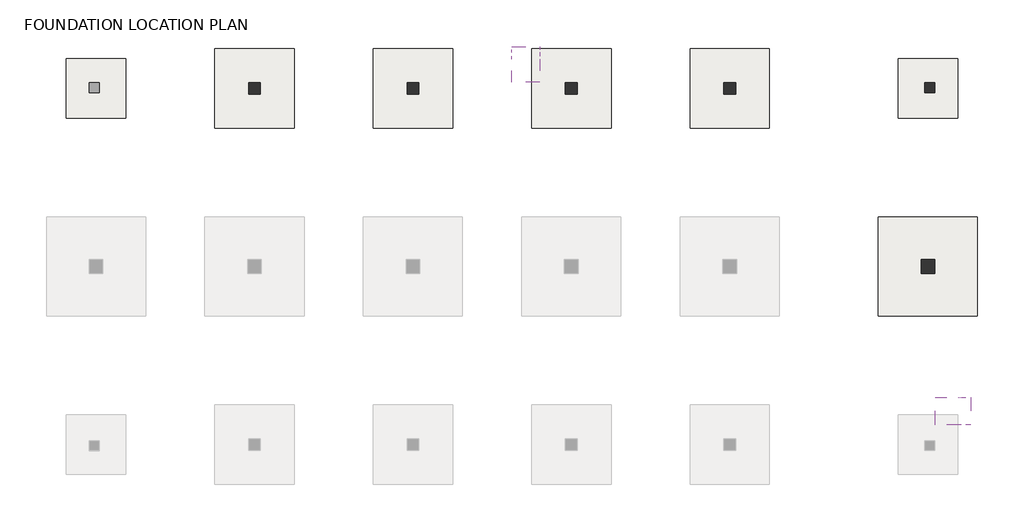
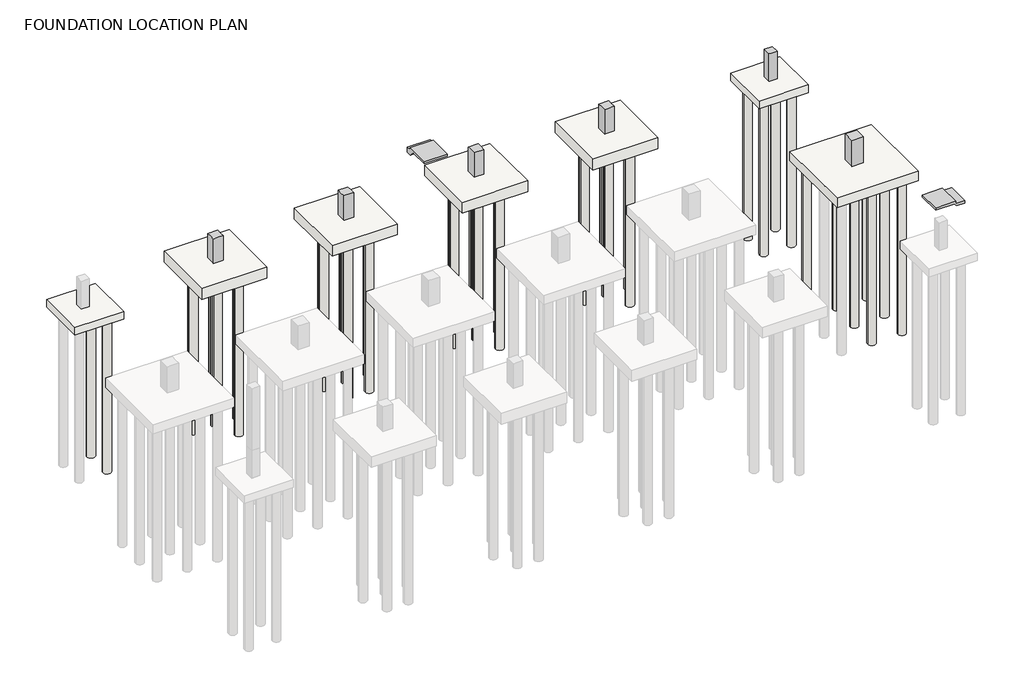
# One storey, part 3 of 3: 48 slabs, 6 columns, 2 proxies.
"""IFC4 building model written with IfcOpenShell, lengths in millimetres."""

import ifcopenshell
import ifcopenshell.guid

model = None  # the IFC model being written
_history = None  # IfcOwnerHistory: only IFC2X3 demands one
_inside = {}  # id of a spatial element -> (the spatial element, [elements in it])
_under = {}  # id of a project, library or spatial element -> (it, [spatial elements below it])
_declared = {}  # id of a project -> (the project, [libraries it declares])
_typed = {}  # id of a type object -> (the type object, [elements of that type])
_made_of = {}  # id of a material, layer set ... -> (it, [elements and type objects made of it])


def new_model(schema):
    """Start an empty IFC model of exactly this schema.

    Asked for "IFC4X3", IfcOpenShell would pick the latest addendum, in which some entities
    have other attributes; the version numbers below select the first issue.
    IFC2X3 requires an IfcOwnerHistory on every rooted entity: one is made here for all.
    """
    global model, _history
    if schema == "IFC4X3":
        model = ifcopenshell.file(schema_version=(4, 3, 0, 0))
    else:
        model = ifcopenshell.file(schema=schema)
    _inside.clear()
    _under.clear()
    _declared.clear()
    _typed.clear()
    _made_of.clear()
    _history = None
    if model.schema == "IFC2X3":
        org = make("IfcOrganization", Name="unknown")
        user = make(
            "IfcPersonAndOrganization",
            ThePerson=make("IfcPerson", FamilyName="unknown"),
            TheOrganization=org,
        )
        app = make(
            "IfcApplication",
            ApplicationDeveloper=org,
            Version="unknown",
            ApplicationFullName="unknown",
            ApplicationIdentifier="unknown",
        )
        _history = make(
            "IfcOwnerHistory",
            OwningUser=user,
            OwningApplication=app,
            ChangeAction="ADDED",
            CreationDate=0,
        )
    return model


def make(cls, **values):
    """One entity of the class cls with the attributes given. An attribute that is None is left unset."""
    return model.create_entity(
        cls, **{name: value for name, value in values.items() if value is not None}
    )


def rooted(cls, **values):
    """An entity with a GlobalId (a new one), such as an element, a storey or a relation."""
    return make(cls, GlobalId=ifcopenshell.guid.new(), OwnerHistory=_history, **values)


def si_unit(unit_type, name, prefix=None):
    """IfcSIUnit, for example si_unit("LENGTHUNIT", "METRE", prefix="MILLI")."""
    return make("IfcSIUnit", UnitType=unit_type, Prefix=prefix, Name=name)


def assignment(units):
    """IfcUnitAssignment: the units of a project."""
    return None if units is None else make("IfcUnitAssignment", Units=units)


def point(xyz):
    """IfcCartesianPoint."""
    return None if xyz is None else make("IfcCartesianPoint", Coordinates=xyz)


def direction(xyz):
    """IfcDirection."""
    return None if xyz is None else make("IfcDirection", DirectionRatios=xyz)


def frame(location, z_axis=None, x_axis=None):
    """IfcAxis2Placement3D, a coordinate frame: its origin and axes. An axis left out is left unset."""
    return make(
        "IfcAxis2Placement3D",
        Location=point(location),
        Axis=direction(z_axis),
        RefDirection=direction(x_axis),
    )


def frame_2d(location, x_axis=None):
    """IfcAxis2Placement2D, a coordinate frame in the plane: its origin and x axis."""
    return make(
        "IfcAxis2Placement2D", Location=point(location), RefDirection=direction(x_axis)
    )


def origin():
    """The frame at (0, 0, 0) with its axes left unset."""
    return frame((0.0, 0.0, 0.0))


def place(relative_to, where):
    """IfcLocalPlacement: puts the frame where relative to a parent placement (None: the world)."""
    return make(
        "IfcLocalPlacement", PlacementRelTo=relative_to, RelativePlacement=where
    )


def context(
    kind, dimensions, precision=None, world=None, true_north=None, identifier=None
):
    """IfcGeometricRepresentationContext, for example the 3D "Model" context."""
    return make(
        "IfcGeometricRepresentationContext",
        ContextIdentifier=identifier,
        ContextType=kind,
        CoordinateSpaceDimension=dimensions,
        Precision=precision,
        WorldCoordinateSystem=world,
        TrueNorth=true_north,
    )


def project(units=None, contexts=None):
    """IfcProject with its units and contexts."""
    return rooted(
        "IfcProject",
        Name="project",
        RepresentationContexts=contexts,
        UnitsInContext=assignment(units),
    )


def spatial(cls, under=None, at=None, **own):
    """A site, building, storey or space (cls), placed at a placement, below another one or the project."""
    s = rooted(cls, ObjectPlacement=at, **own)
    if under is not None:
        _under.setdefault(under.id(), (under, []))[1].append(s)
    return s


def polyline(points):
    """IfcPolyline through the points."""
    return make("IfcPolyline", Points=[point(p) for p in points])


def circle_curve(where, radius):
    """IfcCircle in the frame where."""
    return make("IfcCircle", Position=where, Radius=radius)


def trimmed(basis, trim1, trim2, sense, master):
    """IfcTrimmedCurve: the piece of a basis curve between two trims."""
    return make(
        "IfcTrimmedCurve",
        BasisCurve=basis,
        Trim1=trim1,
        Trim2=trim2,
        SenseAgreement=sense,
        MasterRepresentation=master,
    )


def segment(curve, same_sense, transition):
    """IfcCompositeCurveSegment."""
    return make(
        "IfcCompositeCurveSegment",
        Transition=transition,
        SameSense=same_sense,
        ParentCurve=curve,
    )


def composite_curve(segments, self_intersect=None):
    """IfcCompositeCurve: segments joined end to end."""
    return make("IfcCompositeCurve", Segments=segments, SelfIntersect=self_intersect)


def outline(outer, holes=None, kind="AREA"):
    """IfcArbitraryClosedProfileDef: a profile drawn as a closed curve; with holes, ...WithVoids."""
    if holes is None:
        return make("IfcArbitraryClosedProfileDef", ProfileType=kind, OuterCurve=outer)
    return make(
        "IfcArbitraryProfileDefWithVoids",
        ProfileType=kind,
        OuterCurve=outer,
        InnerCurves=holes,
    )


def extrude(swept, where, along, depth):
    """IfcExtrudedAreaSolid: the profile swept, set in the frame where, extruded along a direction by depth."""
    return make(
        "IfcExtrudedAreaSolid",
        SweptArea=swept,
        Position=where,
        ExtrudedDirection=direction(along),
        Depth=depth,
    )


def faces_of(points, faces, orient=None, outer=None):
    """IfcFace entities. A face is a list of loops; a loop is a list of indices into points, from 0.

    orient and outer hold one flag for each loop. By default every Orientation is true, the
    first loop of a face is its IfcFaceOuterBound and the others are IfcFaceBound.
    """
    made = []
    for i, loops in enumerate(faces):
        bounds = []
        for j, loop in enumerate(loops):
            is_outer = j == 0 if outer is None else outer[i][j]
            bounds.append(
                make(
                    "IfcFaceOuterBound" if is_outer else "IfcFaceBound",
                    Bound=make("IfcPolyLoop", Polygon=[points[k] for k in loop]),
                    Orientation=True if orient is None else orient[i][j],
                )
            )
        made.append(make("IfcFace", Bounds=bounds))
    return made


def faceted_brep(points, faces, orient=None, outer=None, voids=None):
    """IfcFacetedBrep: a solid bounded by flat faces; with voids (closed shells), ...WithVoids."""
    shared = [point(p) for p in points]
    hull = make("IfcClosedShell", CfsFaces=faces_of(shared, faces, orient, outer))
    if voids is None:
        return make("IfcFacetedBrep", Outer=hull)
    return make(
        "IfcFacetedBrepWithVoids",
        Outer=hull,
        Voids=[
            make(cls, CfsFaces=faces_of(shared, fs, o, b)) for cls, fs, o, b in voids
        ],
    )


def shape(context_of_items, identifier, shape_type, items):
    """IfcShapeRepresentation: the items that make up one representation, for example the "Body"."""
    return make(
        "IfcShapeRepresentation",
        ContextOfItems=context_of_items,
        RepresentationIdentifier=identifier,
        RepresentationType=shape_type,
        Items=items,
    )


def source(mapping_origin, context_of_items, identifier, shape_type, items):
    """IfcRepresentationMap: a shape defined once, which mapped items show again and again."""
    return make(
        "IfcRepresentationMap",
        MappingOrigin=mapping_origin,
        MappedRepresentation=shape(context_of_items, identifier, shape_type, items),
    )


def transform(
    local_origin,
    x_axis=None,
    y_axis=None,
    z_axis=None,
    scale=None,
    scale2=None,
    scale3=None,
    uniform=True,
):
    """IfcCartesianTransformationOperator3D, or its non-uniform kind. x_axis, y_axis, z_axis: its Axis1, 2, 3."""
    if uniform:
        return make(
            "IfcCartesianTransformationOperator3D",
            Axis1=direction(x_axis),
            Axis2=direction(y_axis),
            LocalOrigin=point(local_origin),
            Scale=scale,
            Axis3=direction(z_axis),
        )
    return make(
        "IfcCartesianTransformationOperator3DnonUniform",
        Axis1=direction(x_axis),
        Axis2=direction(y_axis),
        LocalOrigin=point(local_origin),
        Scale=scale,
        Axis3=direction(z_axis),
        Scale2=scale2,
        Scale3=scale3,
    )


def mapped(mapping_source, mapping_target):
    """IfcMappedItem: shows the shape of a source again, moved by a transform."""
    return make(
        "IfcMappedItem", MappingSource=mapping_source, MappingTarget=mapping_target
    )


def made_of(thing, what):
    """Note that an element or type object is made of a material, layer set ...; save() writes the relation."""
    if what is not None:
        _made_of.setdefault(what.id(), (what, []))[1].append(thing)
    return thing


def element(
    cls,
    number,
    at=None,
    inside=None,
    cuts=None,
    type_object=None,
    material=None,
    context=None,
    identifier="Body",
    shape_type=None,
    held_by="IfcProductDefinitionShape",
    body=None,
    shapes=None,
    **own,
):
    """One element of the class cls, such as IfcWall. Its Tag is "e" and its number.

    at: its placement. inside: the storey or other place that contains it. cuts: it is an
    opening in that element (IfcRelVoidsElement). A single representation is given by context,
    identifier, shape_type and body (its items); several are given by shapes. held_by: the class
    of the entity that holds the representations. save() writes the other relations.
    """
    e = rooted(cls, Tag="e%d" % number, ObjectPlacement=at, **own)
    if body is not None:
        shapes = [shape(context, identifier, shape_type, body)]
    if shapes is not None:
        e.Representation = make(held_by, Representations=shapes)
    if inside is not None:
        _inside.setdefault(inside.id(), (inside, []))[1].append(e)
    if cuts is not None:
        rooted(
            "IfcRelVoidsElement", RelatingBuildingElement=cuts, RelatedOpeningElement=e
        )
    if type_object is not None:
        _typed.setdefault(type_object.id(), (type_object, []))[1].append(e)
    return made_of(e, material)


def aggregate(whole, parts):
    """IfcRelAggregates: a whole, such as a stair, and the parts it consists of."""
    return rooted("IfcRelAggregates", RelatingObject=whole, RelatedObjects=parts)


def save(model, path):
    """Write the relations noted so far, then the file.

    IfcRelAggregates (storeys below a building ...), IfcRelContainedInSpatialStructure (elements
    in a storey), IfcRelDefinesByType, IfcRelAssociatesMaterial and IfcRelDeclares: one each for
    every whole, place, type object, material and project.
    """
    for whole, parts in _under.values():
        aggregate(whole, parts)
    for where, things in _inside.values():
        rooted(
            "IfcRelContainedInSpatialStructure",
            RelatedElements=things,
            RelatingStructure=where,
        )
    for kind, things in _typed.values():
        rooted("IfcRelDefinesByType", RelatedObjects=things, RelatingType=kind)
    for what, things in _made_of.values():
        rooted("IfcRelAssociatesMaterial", RelatedObjects=things, RelatingMaterial=what)
    for by, libraries in _declared.values():
        rooted("IfcRelDeclares", RelatingContext=by, RelatedDefinitions=libraries)
    model.write(path)


def generic_models_a06d278e(model_context):
    return source(origin(), model_context, "Body", "SweptSolid", [
        extrude(outline(polyline([(599.905241, 43602.1335861), (599.905241, 42370.0), (449.905241, 42370.0), (449.905241, 43520.0), (299.905241, 43670.0), (299.905241, 44170.4893475), (449.905241, 44170.4893475), (449.905241, 43602.1335861), (599.905241, 43602.1335861)])), frame((0.0, 21999.5208589, 0.0), z_axis=(0.0, 1.0, 0.0), x_axis=(0.0, 0.0, 1.0)), (0.0, 0.0, 1.0), 1400.0),
    ])


def generic_models_c40cd3bd(model_context):
    return source(origin(), model_context, "Body", "SweptSolid", [
        extrude(outline(polyline([(40819.5208589, 599.905241), (40819.5208589, 449.905241), (41119.5208589, 449.905241), (41119.5208589, 109.2314637), (40810.1946362, 109.2314637), (40469.5208589, 449.905241), (39319.5208589, 449.905241), (39319.5208589, 599.905241), (40819.5208589, 599.905241)])), frame((21000.0, 0.0, 0.0), z_axis=(1.0, 0.0, 0.0), x_axis=(0.0, 1.0, 0.0)), (0.0, 0.0, 1.0), 1400.0),
    ])


model = new_model("IFC4")

# Units and contexts
model_context = context("Model", 3, world=origin())
ifc_project = project(units=[si_unit("LENGTHUNIT", "METRE", prefix="MILLI")], contexts=[model_context])

# Site, building, storey
site = spatial("IfcSite", under=ifc_project)
building = spatial("IfcBuilding", under=site)
storey = spatial("IfcBuildingStorey", under=building, Name="FOUNDATION LOCATION PLAN", Elevation=-1699.994759)

# Proxies
placement = place(None, origin())
generic_models_shape = generic_models_a06d278e(model_context)
element("IfcBuildingElementProxy", 1, Name="벽 5 : 벽 1", ObjectType="벽 5 : 벽 1", at=placement, inside=storey, context=model_context, shape_type="MappedRepresentation", body=[
    mapped(generic_models_shape, transform((0.0, 0.0, 0.0), x_axis=(1.0, 0.0, 0.0), y_axis=(0.0, 1.0, 0.0), z_axis=(0.0, 0.0, 1.0))),
])
generic_models_2_shape = generic_models_c40cd3bd(model_context)
element("IfcBuildingElementProxy", 2, Name="벽 1 : 벽 1", ObjectType="벽 1 : 벽 1", at=placement, inside=storey, context=model_context, shape_type="MappedRepresentation", body=[
    mapped(generic_models_2_shape, transform((0.0, 0.0, 0.0), x_axis=(1.0, 0.0, 0.0), y_axis=(0.0, 1.0, 0.0), z_axis=(0.0, 0.0, 1.0))),
])

# Columns
element("IfcColumn", 3, ObjectType="Concrete-Rectangular-Column_R1 : CLS111_RC COLUMN_UG_C1", at=placement, inside=storey, context=model_context, shape_type="Brep", body=[
    faceted_brep([(41850.0, 39299.5208589, -1199.994759), (42350.0, 39299.5208589, -1199.994759), (42350.0, 38799.5208589, -1199.994759), (41850.0, 38799.5208589, -1199.994759), (41850.0, 39299.5208589, 600.005241), (42350.0, 39299.5208589, 600.005241), (41850.0, 38799.5208589, 450.005241), (41850.0, 38799.5208589, 600.005241), (41850.0, 38999.7368538, 600.005241), (42350.0, 38799.5208589, 600.005241), (42000.0, 38799.5208589, 600.005241)], [[[0, 1, 2, 3]], [[1, 0, 4, 5]], [[0, 3, 6, 7, 8, 4]], [[3, 2, 9, 10, 7, 6]], [[2, 1, 5, 9]], [[5, 4, 8, 7, 10, 9]]]),
])
element("IfcColumn", 4, ObjectType="Concrete-Rectangular-Column_R1 : CLS111_RC COLUMN_UG_C3", at=placement, inside=storey, context=model_context, shape_type="Brep", body=[
    faceted_brep([(41650.0, 30349.5208589, -1099.994759), (42350.0, 30349.5208589, -1099.994759), (42350.0, 29649.5208589, -1099.994759), (41650.0, 29649.5208589, -1099.994759), (41650.0, 30349.5208589, 450.005241), (41650.0, 30349.5208589, 600.005241), (42000.0, 30349.5208589, 600.005241), (42350.0, 30349.5208589, 600.005241), (41650.0, 29649.5208589, 450.005241), (41650.0, 29649.5208589, 600.005241), (42350.0, 29649.5208589, 600.005241)], [[[0, 1, 2, 3]], [[1, 0, 4, 5, 6, 7]], [[0, 3, 8, 9, 5, 4]], [[3, 2, 10, 9, 8]], [[2, 1, 7, 10]], [[5, 9, 10, 7, 6]]]),
])
element("IfcColumn", 5, ObjectType="Concrete-Rectangular-Column_R1 : CLS111_RC COLUMN_UG_C2", at=placement, inside=storey, context=model_context, shape_type="Brep", body=[
    faceted_brep([(7700.0, 39299.7368538, -999.994759), (8300.0, 39299.7368538, -999.994759), (8300.0, 38699.7368538, -999.994759), (7700.0, 38699.7368538, -999.994759), (7700.0, 39299.7368538, 600.005241), (8300.0, 39299.7368538, 600.005241), (8300.0, 39299.5208589, 600.005241), (8300.0, 38999.7634659, 600.005241), (8300.0, 38699.7368538, 600.005241), (8300.0, 38699.7368538, 450.005241), (8100.0, 38699.7368538, 600.005241), (7700.0, 38699.7368538, 600.005241), (7700.0, 38699.7368538, 450.005241), (7700.0, 38699.7368538, 0.005241), (7700.0, 38999.7368538, 600.005241), (7700.0, 39299.5208589, 600.005241)], [[[0, 1, 2, 3]], [[1, 0, 4, 5]], [[2, 1, 5, 6, 7, 8, 9]], [[3, 2, 9, 8, 10, 11, 12, 13]], [[0, 3, 13, 12, 11, 14, 15, 4]], [[5, 4, 15, 14, 11, 10, 8, 7, 6]]]),
])
element("IfcColumn", 6, ObjectType="Concrete-Rectangular-Column_R1 : CLS111_RC COLUMN_UG_C2", at=placement, inside=storey, context=model_context, shape_type="Brep", body=[
    faceted_brep([(15700.0, 39299.7368538, -999.994759), (16300.0, 39299.7368538, -999.994759), (16300.0, 38699.7368538, -999.994759), (15700.0, 38699.7368538, -999.994759), (15700.0, 39299.7368538, 600.005241), (16300.0, 39299.7368538, 600.005241), (16300.0, 39299.5208589, 600.005241), (16300.0, 38999.7368538, 600.005241), (16300.0, 38699.7368538, 600.005241), (16300.0, 38699.7368538, 450.005241), (16200.0, 38699.7368538, 600.005241), (15800.0, 38699.7368538, 600.005241), (15700.0, 38699.7368538, 600.005241), (15700.0, 38699.7368538, 450.005241), (15700.0, 38999.7634659, 600.005241), (15700.0, 39299.5208589, 600.005241)], [[[0, 1, 2, 3]], [[1, 0, 4, 5]], [[2, 1, 5, 6, 7, 8, 9]], [[3, 2, 9, 8, 10, 11, 12, 13]], [[0, 3, 13, 12, 14, 15, 4]], [[5, 4, 15, 14, 12, 11, 10, 8, 7, 6]]]),
])
element("IfcColumn", 7, ObjectType="Concrete-Rectangular-Column_R1 : CLS111_RC COLUMN_UG_C2", at=placement, inside=storey, context=model_context, shape_type="Brep", body=[
    faceted_brep([(23700.0, 39299.7368538, -999.994759), (24300.0, 39299.7368538, -999.994759), (24300.0, 38699.7368538, -999.994759), (23700.0, 38699.7368538, -999.994759), (23700.0, 39299.7368538, 600.005241), (24300.0, 39299.7368538, 600.005241), (24300.0, 39299.5208589, 600.005241), (24300.0, 38999.7368538, 600.005241), (24300.0, 38699.7368538, 600.005241), (24300.0, 38699.7368538, 450.005241), (24200.0, 38699.7368538, 600.005241), (23800.0, 38699.7368538, 600.005241), (23700.0, 38699.7368538, 600.005241), (23700.0, 38699.7368538, 450.005241), (23700.0, 38999.7368538, 600.005241), (23700.0, 39299.5208589, 600.005241)], [[[0, 1, 2, 3]], [[1, 0, 4, 5]], [[2, 1, 5, 6, 7, 8, 9]], [[3, 2, 9, 8, 10, 11, 12, 13]], [[0, 3, 13, 12, 14, 15, 4]], [[5, 4, 15, 14, 12, 11, 10, 8, 7, 6]]]),
])
element("IfcColumn", 8, ObjectType="Concrete-Rectangular-Column_R1 : CLS111_RC COLUMN_UG_C2", at=placement, inside=storey, context=model_context, shape_type="Brep", body=[
    faceted_brep([(31700.0, 39299.7368538, -999.994759), (32300.0, 39299.7368538, -999.994759), (32300.0, 38699.7368538, -999.994759), (31700.0, 38699.7368538, -999.994759), (31700.0, 39299.7368538, 600.005241), (32300.0, 39299.7368538, 600.005241), (32300.0, 39299.5208589, 600.005241), (32300.0, 38999.7368538, 600.005241), (32300.0, 38699.7368538, 600.005241), (32300.0, 38699.7368538, 450.005241), (32200.0, 38699.7368538, 600.005241), (31800.0, 38699.7368538, 600.005241), (31700.0, 38699.7368538, 600.005241), (31700.0, 38699.7368538, 450.005241), (31700.0, 38999.7368538, 600.005241), (31700.0, 39299.5208589, 600.005241)], [[[0, 1, 2, 3]], [[1, 0, 4, 5]], [[2, 1, 5, 6, 7, 8, 9]], [[3, 2, 9, 8, 10, 11, 12, 13]], [[0, 3, 13, 12, 14, 15, 4]], [[5, 4, 15, 14, 12, 11, 10, 8, 7, 6]]]),
])

# Slabs
element("IfcSlab", 9, ObjectType="Footing-Rectangular_R1 : FTS301_Footing-Rectangular_3000x3000x500_F1", at=placement, inside=storey, context=model_context, shape_type="SweptSolid", body=[
    extrude(outline(polyline([(1500.0, 40499.7368538), (1500.0, 37499.7368538), (-1500.0, 37499.7368538), (-1500.0, 40499.7368538), (1500.0, 40499.7368538)])), frame((0.0, 0.0, -1699.994759), z_axis=(0.0, 0.0, 1.0), x_axis=(1.0, 0.0, 0.0)), (0.0, 0.0, 1.0), 500.0),
])
element("IfcSlab", 10, ObjectType="Footing-Rectangular_R1 : FTS301_Footing-Rectangular_3000x3000x500_F1", at=placement, inside=storey, context=model_context, shape_type="SweptSolid", body=[
    extrude(outline(polyline([(43500.0, 40499.7368538), (43500.0, 37499.7368538), (40500.0, 37499.7368538), (40500.0, 40499.7368538), (43500.0, 40499.7368538)])), frame((0.0, 0.0, -1699.994759), z_axis=(0.0, 0.0, 1.0), x_axis=(1.0, 0.0, 0.0)), (0.0, 0.0, 1.0), 500.0),
])
element("IfcSlab", 11, ObjectType="Footing-Rectangular_R1 : FTS301_Footing-Rectangular_4000x4000x700_F2", at=placement, inside=storey, context=model_context, shape_type="SweptSolid", body=[
    extrude(outline(polyline([(10000.0, 40999.7368538), (10000.0, 36999.7368538), (6000.0, 36999.7368538), (6000.0, 40999.7368538), (10000.0, 40999.7368538)])), frame((0.0, 0.0, -1699.994759), z_axis=(0.0, 0.0, 1.0), x_axis=(1.0, 0.0, 0.0)), (0.0, 0.0, 1.0), 700.0),
])
element("IfcSlab", 12, ObjectType="Footing-Rectangular_R1 : FTS301_Footing-Rectangular_4000x4000x700_F2", at=placement, inside=storey, context=model_context, shape_type="SweptSolid", body=[
    extrude(outline(polyline([(18000.0, 40999.7368538), (18000.0, 36999.7368538), (14000.0, 36999.7368538), (14000.0, 40999.7368538), (18000.0, 40999.7368538)])), frame((0.0, 0.0, -1699.994759), z_axis=(0.0, 0.0, 1.0), x_axis=(1.0, 0.0, 0.0)), (0.0, 0.0, 1.0), 700.0),
])
element("IfcSlab", 13, ObjectType="Footing-Rectangular_R1 : FTS301_Footing-Rectangular_4000x4000x700_F2", at=placement, inside=storey, context=model_context, shape_type="SweptSolid", body=[
    extrude(outline(polyline([(26000.0, 40999.7368538), (26000.0, 36999.7368538), (22000.0, 36999.7368538), (22000.0, 40999.7368538), (26000.0, 40999.7368538)])), frame((0.0, 0.0, -1699.994759), z_axis=(0.0, 0.0, 1.0), x_axis=(1.0, 0.0, 0.0)), (0.0, 0.0, 1.0), 700.0),
])
element("IfcSlab", 14, ObjectType="Footing-Rectangular_R1 : FTS301_Footing-Rectangular_4000x4000x700_F2", at=placement, inside=storey, context=model_context, shape_type="SweptSolid", body=[
    extrude(outline(polyline([(34000.0, 40999.7368538), (34000.0, 36999.7368538), (30000.0, 36999.7368538), (30000.0, 40999.7368538), (34000.0, 40999.7368538)])), frame((0.0, 0.0, -1699.994759), z_axis=(0.0, 0.0, 1.0), x_axis=(1.0, 0.0, 0.0)), (0.0, 0.0, 1.0), 700.0),
])
element("IfcSlab", 15, ObjectType="Footing-Rectangular_R1 : FTS301_Footing-Rectangular_5000x5000x600_F3", at=placement, inside=storey, context=model_context, shape_type="SweptSolid", body=[
    extrude(outline(polyline([(44500.0, 32499.5208589), (44500.0, 27499.5208589), (39500.0, 27499.5208589), (39500.0, 32499.5208589), (44500.0, 32499.5208589)])), frame((0.0, 0.0, -1699.994759), z_axis=(0.0, 0.0, 1.0), x_axis=(1.0, 0.0, 0.0)), (0.0, 0.0, 1.0), 600.0),
])
element("IfcSlab", 16, ObjectType="HEC_PILE : FTPS102_D500", at=placement, inside=storey, context=model_context, shape_type="SweptSolid", body=[
    extrude(outline(composite_curve([segment(trimmed(circle_curve(frame_2d((850.0, 39849.5208589)), 250.0), [point((600.0, 39849.5208589))], [point((1100.0, 39849.5208589))], False, "CARTESIAN"), True, "CONTINUOUS"), segment(trimmed(circle_curve(frame_2d((850.0, 39849.5208589)), 250.0), [point((1100.0, 39849.5208589))], [point((600.0, 39849.5208589))], False, "CARTESIAN"), True, "CONTINUOUS")], self_intersect=False)), frame((0.0, 0.0, -11749.994759), z_axis=(0.0, 0.0, 1.0), x_axis=(1.0, 0.0, 0.0)), (0.0, 0.0, 1.0), 10150.0),
])
element("IfcSlab", 17, ObjectType="HEC_PILE : FTPS102_D500", at=placement, inside=storey, context=model_context, shape_type="SweptSolid", body=[
    extrude(outline(composite_curve([segment(trimmed(circle_curve(frame_2d((41150.0, 39849.5208589)), 250.0), [point((41400.0, 39849.5208589))], [point((40900.0, 39849.5208589))], False, "CARTESIAN"), True, "CONTINUOUS"), segment(trimmed(circle_curve(frame_2d((41150.0, 39849.5208589)), 250.0), [point((40900.0, 39849.5208589))], [point((41400.0, 39849.5208589))], False, "CARTESIAN"), True, "CONTINUOUS")], self_intersect=False)), frame((0.0, 0.0, -11749.994759), z_axis=(0.0, 0.0, 1.0), x_axis=(1.0, 0.0, 0.0)), (0.0, 0.0, 1.0), 10150.0),
])
element("IfcSlab", 18, ObjectType="HEC_PILE : FTPS102_D500", at=placement, inside=storey, context=model_context, shape_type="SweptSolid", body=[
    extrude(outline(composite_curve([segment(trimmed(circle_curve(frame_2d((42850.0, 39849.5208589)), 250.0), [point((42600.0, 39849.5208589))], [point((43100.0, 39849.5208589))], False, "CARTESIAN"), True, "CONTINUOUS"), segment(trimmed(circle_curve(frame_2d((42850.0, 39849.5208589)), 250.0), [point((43100.0, 39849.5208589))], [point((42600.0, 39849.5208589))], False, "CARTESIAN"), True, "CONTINUOUS")], self_intersect=False)), frame((0.0, 0.0, -11749.994759), z_axis=(0.0, 0.0, 1.0), x_axis=(1.0, 0.0, 0.0)), (0.0, 0.0, 1.0), 10150.0),
])
element("IfcSlab", 19, ObjectType="HEC_PILE : FTPS102_D500", at=placement, inside=storey, context=model_context, shape_type="SweptSolid", body=[
    extrude(outline(composite_curve([segment(trimmed(circle_curve(frame_2d((41150.0, 38149.5208589)), 250.0), [point((41400.0, 38149.5208589))], [point((40900.0, 38149.5208589))], False, "CARTESIAN"), True, "CONTINUOUS"), segment(trimmed(circle_curve(frame_2d((41150.0, 38149.5208589)), 250.0), [point((40900.0, 38149.5208589))], [point((41400.0, 38149.5208589))], False, "CARTESIAN"), True, "CONTINUOUS")], self_intersect=False)), frame((0.0, 0.0, -11749.994759), z_axis=(0.0, 0.0, 1.0), x_axis=(1.0, 0.0, 0.0)), (0.0, 0.0, 1.0), 10150.0),
])
element("IfcSlab", 20, ObjectType="HEC_PILE : FTPS102_D500", at=placement, inside=storey, context=model_context, shape_type="SweptSolid", body=[
    extrude(outline(composite_curve([segment(trimmed(circle_curve(frame_2d((42850.0, 38149.5208589)), 250.0), [point((42600.0, 38149.5208589))], [point((43100.0, 38149.5208589))], False, "CARTESIAN"), True, "CONTINUOUS"), segment(trimmed(circle_curve(frame_2d((42850.0, 38149.5208589)), 250.0), [point((43100.0, 38149.5208589))], [point((42600.0, 38149.5208589))], False, "CARTESIAN"), True, "CONTINUOUS")], self_intersect=False)), frame((0.0, 0.0, -11749.994759), z_axis=(0.0, 0.0, 1.0), x_axis=(1.0, 0.0, 0.0)), (0.0, 0.0, 1.0), 10150.0),
])
element("IfcSlab", 21, ObjectType="HEC_PILE : FTPS102_D500", at=placement, inside=storey, context=model_context, shape_type="SweptSolid", body=[
    extrude(outline(composite_curve([segment(trimmed(circle_curve(frame_2d((31350.0, 37649.5208589)), 250.0), [point((31600.0, 37649.5208589))], [point((31100.0, 37649.5208589))], False, "CARTESIAN"), True, "CONTINUOUS"), segment(trimmed(circle_curve(frame_2d((31350.0, 37649.5208589)), 250.0), [point((31100.0, 37649.5208589))], [point((31600.0, 37649.5208589))], False, "CARTESIAN"), True, "CONTINUOUS")], self_intersect=False)), frame((0.0, 0.0, -11749.994759), z_axis=(0.0, 0.0, 1.0), x_axis=(1.0, 0.0, 0.0)), (0.0, 0.0, 1.0), 10150.0),
])
element("IfcSlab", 22, ObjectType="HEC_PILE : FTPS102_D500", at=placement, inside=storey, context=model_context, shape_type="SweptSolid", body=[
    extrude(outline(composite_curve([segment(trimmed(circle_curve(frame_2d((32650.0, 37649.5208589)), 250.0), [point((32400.0, 37649.5208589))], [point((32900.0, 37649.5208589))], False, "CARTESIAN"), True, "CONTINUOUS"), segment(trimmed(circle_curve(frame_2d((32650.0, 37649.5208589)), 250.0), [point((32900.0, 37649.5208589))], [point((32400.0, 37649.5208589))], False, "CARTESIAN"), True, "CONTINUOUS")], self_intersect=False)), frame((0.0, 0.0, -11749.994759), z_axis=(0.0, 0.0, 1.0), x_axis=(1.0, 0.0, 0.0)), (0.0, 0.0, 1.0), 10150.0),
])
element("IfcSlab", 23, ObjectType="HEC_PILE : FTPS102_D500", at=placement, inside=storey, context=model_context, shape_type="SweptSolid", body=[
    extrude(outline(composite_curve([segment(trimmed(circle_curve(frame_2d((30650.0, 38999.5208589)), 250.0), [point((30900.0, 38999.5208589))], [point((30400.0, 38999.5208589))], False, "CARTESIAN"), True, "CONTINUOUS"), segment(trimmed(circle_curve(frame_2d((30650.0, 38999.5208589)), 250.0), [point((30400.0, 38999.5208589))], [point((30900.0, 38999.5208589))], False, "CARTESIAN"), True, "CONTINUOUS")], self_intersect=False)), frame((0.0, 0.0, -11749.994759), z_axis=(0.0, 0.0, 1.0), x_axis=(1.0, 0.0, 0.0)), (0.0, 0.0, 1.0), 10150.0),
])
element("IfcSlab", 24, ObjectType="HEC_PILE : FTPS102_D500", at=placement, inside=storey, context=model_context, shape_type="SweptSolid", body=[
    extrude(outline(composite_curve([segment(trimmed(circle_curve(frame_2d((32000.0, 38999.5208589)), 250.0), [point((32250.0, 38999.5208589))], [point((31750.0, 38999.5208589))], False, "CARTESIAN"), True, "CONTINUOUS"), segment(trimmed(circle_curve(frame_2d((32000.0, 38999.5208589)), 250.0), [point((31750.0, 38999.5208589))], [point((32250.0, 38999.5208589))], False, "CARTESIAN"), True, "CONTINUOUS")], self_intersect=False)), frame((0.0, 0.0, -11749.994759), z_axis=(0.0, 0.0, 1.0), x_axis=(1.0, 0.0, 0.0)), (0.0, 0.0, 1.0), 10150.0),
])
element("IfcSlab", 25, ObjectType="HEC_PILE : FTPS102_D500", at=placement, inside=storey, context=model_context, shape_type="SweptSolid", body=[
    extrude(outline(composite_curve([segment(trimmed(circle_curve(frame_2d((33350.0, 38999.5208589)), 250.0), [point((33100.0, 38999.5208589))], [point((33600.0, 38999.5208589))], False, "CARTESIAN"), True, "CONTINUOUS"), segment(trimmed(circle_curve(frame_2d((33350.0, 38999.5208589)), 250.0), [point((33600.0, 38999.5208589))], [point((33100.0, 38999.5208589))], False, "CARTESIAN"), True, "CONTINUOUS")], self_intersect=False)), frame((0.0, 0.0, -11749.994759), z_axis=(0.0, 0.0, 1.0), x_axis=(1.0, 0.0, 0.0)), (0.0, 0.0, 1.0), 10150.0),
])
element("IfcSlab", 26, ObjectType="HEC_PILE : FTPS102_D500", at=placement, inside=storey, context=model_context, shape_type="SweptSolid", body=[
    extrude(outline(composite_curve([segment(trimmed(circle_curve(frame_2d((31350.0, 40349.5208589)), 250.0), [point((31600.0, 40349.5208589))], [point((31100.0, 40349.5208589))], False, "CARTESIAN"), True, "CONTINUOUS"), segment(trimmed(circle_curve(frame_2d((31350.0, 40349.5208589)), 250.0), [point((31100.0, 40349.5208589))], [point((31600.0, 40349.5208589))], False, "CARTESIAN"), True, "CONTINUOUS")], self_intersect=False)), frame((0.0, 0.0, -11749.994759), z_axis=(0.0, 0.0, 1.0), x_axis=(1.0, 0.0, 0.0)), (0.0, 0.0, 1.0), 10150.0),
])
element("IfcSlab", 27, ObjectType="HEC_PILE : FTPS102_D500", at=placement, inside=storey, context=model_context, shape_type="SweptSolid", body=[
    extrude(outline(composite_curve([segment(trimmed(circle_curve(frame_2d((32650.0, 40349.5208589)), 250.0), [point((32400.0, 40349.5208589))], [point((32900.0, 40349.5208589))], False, "CARTESIAN"), True, "CONTINUOUS"), segment(trimmed(circle_curve(frame_2d((32650.0, 40349.5208589)), 250.0), [point((32900.0, 40349.5208589))], [point((32400.0, 40349.5208589))], False, "CARTESIAN"), True, "CONTINUOUS")], self_intersect=False)), frame((0.0, 0.0, -11749.994759), z_axis=(0.0, 0.0, 1.0), x_axis=(1.0, 0.0, 0.0)), (0.0, 0.0, 1.0), 10150.0),
])
element("IfcSlab", 28, ObjectType="HEC_PILE : FTPS102_D500", at=placement, inside=storey, context=model_context, shape_type="SweptSolid", body=[
    extrude(outline(composite_curve([segment(trimmed(circle_curve(frame_2d((23350.0, 37649.5208589)), 250.0), [point((23600.0, 37649.5208589))], [point((23100.0, 37649.5208589))], False, "CARTESIAN"), True, "CONTINUOUS"), segment(trimmed(circle_curve(frame_2d((23350.0, 37649.5208589)), 250.0), [point((23100.0, 37649.5208589))], [point((23600.0, 37649.5208589))], False, "CARTESIAN"), True, "CONTINUOUS")], self_intersect=False)), frame((0.0, 0.0, -11749.994759), z_axis=(0.0, 0.0, 1.0), x_axis=(1.0, 0.0, 0.0)), (0.0, 0.0, 1.0), 10150.0),
])
element("IfcSlab", 29, ObjectType="HEC_PILE : FTPS102_D500", at=placement, inside=storey, context=model_context, shape_type="SweptSolid", body=[
    extrude(outline(composite_curve([segment(trimmed(circle_curve(frame_2d((24650.0, 37649.5208589)), 250.0), [point((24400.0, 37649.5208589))], [point((24900.0, 37649.5208589))], False, "CARTESIAN"), True, "CONTINUOUS"), segment(trimmed(circle_curve(frame_2d((24650.0, 37649.5208589)), 250.0), [point((24900.0, 37649.5208589))], [point((24400.0, 37649.5208589))], False, "CARTESIAN"), True, "CONTINUOUS")], self_intersect=False)), frame((0.0, 0.0, -11749.994759), z_axis=(0.0, 0.0, 1.0), x_axis=(1.0, 0.0, 0.0)), (0.0, 0.0, 1.0), 10150.0),
])
element("IfcSlab", 30, ObjectType="HEC_PILE : FTPS102_D500", at=placement, inside=storey, context=model_context, shape_type="SweptSolid", body=[
    extrude(outline(composite_curve([segment(trimmed(circle_curve(frame_2d((22650.0, 38999.5208589)), 250.0), [point((22900.0, 38999.5208589))], [point((22400.0, 38999.5208589))], False, "CARTESIAN"), True, "CONTINUOUS"), segment(trimmed(circle_curve(frame_2d((22650.0, 38999.5208589)), 250.0), [point((22400.0, 38999.5208589))], [point((22900.0, 38999.5208589))], False, "CARTESIAN"), True, "CONTINUOUS")], self_intersect=False)), frame((0.0, 0.0, -11749.994759), z_axis=(0.0, 0.0, 1.0), x_axis=(1.0, 0.0, 0.0)), (0.0, 0.0, 1.0), 10150.0),
])
element("IfcSlab", 31, ObjectType="HEC_PILE : FTPS102_D500", at=placement, inside=storey, context=model_context, shape_type="SweptSolid", body=[
    extrude(outline(composite_curve([segment(trimmed(circle_curve(frame_2d((24000.0, 38999.5208589)), 250.0), [point((24250.0, 38999.5208589))], [point((23750.0, 38999.5208589))], False, "CARTESIAN"), True, "CONTINUOUS"), segment(trimmed(circle_curve(frame_2d((24000.0, 38999.5208589)), 250.0), [point((23750.0, 38999.5208589))], [point((24250.0, 38999.5208589))], False, "CARTESIAN"), True, "CONTINUOUS")], self_intersect=False)), frame((0.0, 0.0, -11749.994759), z_axis=(0.0, 0.0, 1.0), x_axis=(1.0, 0.0, 0.0)), (0.0, 0.0, 1.0), 10150.0),
])
element("IfcSlab", 32, ObjectType="HEC_PILE : FTPS102_D500", at=placement, inside=storey, context=model_context, shape_type="SweptSolid", body=[
    extrude(outline(composite_curve([segment(trimmed(circle_curve(frame_2d((25350.0, 38999.5208589)), 250.0), [point((25100.0, 38999.5208589))], [point((25600.0, 38999.5208589))], False, "CARTESIAN"), True, "CONTINUOUS"), segment(trimmed(circle_curve(frame_2d((25350.0, 38999.5208589)), 250.0), [point((25600.0, 38999.5208589))], [point((25100.0, 38999.5208589))], False, "CARTESIAN"), True, "CONTINUOUS")], self_intersect=False)), frame((0.0, 0.0, -11749.994759), z_axis=(0.0, 0.0, 1.0), x_axis=(1.0, 0.0, 0.0)), (0.0, 0.0, 1.0), 10150.0),
])
element("IfcSlab", 33, ObjectType="HEC_PILE : FTPS102_D500", at=placement, inside=storey, context=model_context, shape_type="SweptSolid", body=[
    extrude(outline(composite_curve([segment(trimmed(circle_curve(frame_2d((23350.0, 40349.5208589)), 250.0), [point((23600.0, 40349.5208589))], [point((23100.0, 40349.5208589))], False, "CARTESIAN"), True, "CONTINUOUS"), segment(trimmed(circle_curve(frame_2d((23350.0, 40349.5208589)), 250.0), [point((23100.0, 40349.5208589))], [point((23600.0, 40349.5208589))], False, "CARTESIAN"), True, "CONTINUOUS")], self_intersect=False)), frame((0.0, 0.0, -11749.994759), z_axis=(0.0, 0.0, 1.0), x_axis=(1.0, 0.0, 0.0)), (0.0, 0.0, 1.0), 10150.0),
])
element("IfcSlab", 34, ObjectType="HEC_PILE : FTPS102_D500", at=placement, inside=storey, context=model_context, shape_type="SweptSolid", body=[
    extrude(outline(composite_curve([segment(trimmed(circle_curve(frame_2d((24650.0, 40349.5208589)), 250.0), [point((24400.0, 40349.5208589))], [point((24900.0, 40349.5208589))], False, "CARTESIAN"), True, "CONTINUOUS"), segment(trimmed(circle_curve(frame_2d((24650.0, 40349.5208589)), 250.0), [point((24900.0, 40349.5208589))], [point((24400.0, 40349.5208589))], False, "CARTESIAN"), True, "CONTINUOUS")], self_intersect=False)), frame((0.0, 0.0, -11749.994759), z_axis=(0.0, 0.0, 1.0), x_axis=(1.0, 0.0, 0.0)), (0.0, 0.0, 1.0), 10150.0),
])
element("IfcSlab", 35, ObjectType="HEC_PILE : FTPS102_D500", at=placement, inside=storey, context=model_context, shape_type="SweptSolid", body=[
    extrude(outline(composite_curve([segment(trimmed(circle_curve(frame_2d((15350.0, 37649.5208589)), 250.0), [point((15600.0, 37649.5208589))], [point((15100.0, 37649.5208589))], False, "CARTESIAN"), True, "CONTINUOUS"), segment(trimmed(circle_curve(frame_2d((15350.0, 37649.5208589)), 250.0), [point((15100.0, 37649.5208589))], [point((15600.0, 37649.5208589))], False, "CARTESIAN"), True, "CONTINUOUS")], self_intersect=False)), frame((0.0, 0.0, -11749.994759), z_axis=(0.0, 0.0, 1.0), x_axis=(1.0, 0.0, 0.0)), (0.0, 0.0, 1.0), 10150.0),
])
element("IfcSlab", 36, ObjectType="HEC_PILE : FTPS102_D500", at=placement, inside=storey, context=model_context, shape_type="SweptSolid", body=[
    extrude(outline(composite_curve([segment(trimmed(circle_curve(frame_2d((16650.0, 37649.5208589)), 250.0), [point((16400.0, 37649.5208589))], [point((16900.0, 37649.5208589))], False, "CARTESIAN"), True, "CONTINUOUS"), segment(trimmed(circle_curve(frame_2d((16650.0, 37649.5208589)), 250.0), [point((16900.0, 37649.5208589))], [point((16400.0, 37649.5208589))], False, "CARTESIAN"), True, "CONTINUOUS")], self_intersect=False)), frame((0.0, 0.0, -11749.994759), z_axis=(0.0, 0.0, 1.0), x_axis=(1.0, 0.0, 0.0)), (0.0, 0.0, 1.0), 10150.0),
])
element("IfcSlab", 37, ObjectType="HEC_PILE : FTPS102_D500", at=placement, inside=storey, context=model_context, shape_type="SweptSolid", body=[
    extrude(outline(composite_curve([segment(trimmed(circle_curve(frame_2d((14650.0, 38999.5208589)), 250.0), [point((14900.0, 38999.5208589))], [point((14400.0, 38999.5208589))], False, "CARTESIAN"), True, "CONTINUOUS"), segment(trimmed(circle_curve(frame_2d((14650.0, 38999.5208589)), 250.0), [point((14400.0, 38999.5208589))], [point((14900.0, 38999.5208589))], False, "CARTESIAN"), True, "CONTINUOUS")], self_intersect=False)), frame((0.0, 0.0, -11749.994759), z_axis=(0.0, 0.0, 1.0), x_axis=(1.0, 0.0, 0.0)), (0.0, 0.0, 1.0), 10150.0),
])
element("IfcSlab", 38, ObjectType="HEC_PILE : FTPS102_D500", at=placement, inside=storey, context=model_context, shape_type="SweptSolid", body=[
    extrude(outline(composite_curve([segment(trimmed(circle_curve(frame_2d((16000.0, 38999.5208589)), 250.0), [point((16250.0, 38999.5208589))], [point((15750.0, 38999.5208589))], False, "CARTESIAN"), True, "CONTINUOUS"), segment(trimmed(circle_curve(frame_2d((16000.0, 38999.5208589)), 250.0), [point((15750.0, 38999.5208589))], [point((16250.0, 38999.5208589))], False, "CARTESIAN"), True, "CONTINUOUS")], self_intersect=False)), frame((0.0, 0.0, -11749.994759), z_axis=(0.0, 0.0, 1.0), x_axis=(1.0, 0.0, 0.0)), (0.0, 0.0, 1.0), 10150.0),
])
element("IfcSlab", 39, ObjectType="HEC_PILE : FTPS102_D500", at=placement, inside=storey, context=model_context, shape_type="SweptSolid", body=[
    extrude(outline(composite_curve([segment(trimmed(circle_curve(frame_2d((17350.0, 38999.5208589)), 250.0), [point((17100.0, 38999.5208589))], [point((17600.0, 38999.5208589))], False, "CARTESIAN"), True, "CONTINUOUS"), segment(trimmed(circle_curve(frame_2d((17350.0, 38999.5208589)), 250.0), [point((17600.0, 38999.5208589))], [point((17100.0, 38999.5208589))], False, "CARTESIAN"), True, "CONTINUOUS")], self_intersect=False)), frame((0.0, 0.0, -11749.994759), z_axis=(0.0, 0.0, 1.0), x_axis=(1.0, 0.0, 0.0)), (0.0, 0.0, 1.0), 10150.0),
])
element("IfcSlab", 40, ObjectType="HEC_PILE : FTPS102_D500", at=placement, inside=storey, context=model_context, shape_type="SweptSolid", body=[
    extrude(outline(composite_curve([segment(trimmed(circle_curve(frame_2d((15350.0, 40349.5208589)), 250.0), [point((15600.0, 40349.5208589))], [point((15100.0, 40349.5208589))], False, "CARTESIAN"), True, "CONTINUOUS"), segment(trimmed(circle_curve(frame_2d((15350.0, 40349.5208589)), 250.0), [point((15100.0, 40349.5208589))], [point((15600.0, 40349.5208589))], False, "CARTESIAN"), True, "CONTINUOUS")], self_intersect=False)), frame((0.0, 0.0, -11749.994759), z_axis=(0.0, 0.0, 1.0), x_axis=(1.0, 0.0, 0.0)), (0.0, 0.0, 1.0), 10150.0),
])
element("IfcSlab", 41, ObjectType="HEC_PILE : FTPS102_D500", at=placement, inside=storey, context=model_context, shape_type="SweptSolid", body=[
    extrude(outline(composite_curve([segment(trimmed(circle_curve(frame_2d((16650.0, 40349.5208589)), 250.0), [point((16400.0, 40349.5208589))], [point((16900.0, 40349.5208589))], False, "CARTESIAN"), True, "CONTINUOUS"), segment(trimmed(circle_curve(frame_2d((16650.0, 40349.5208589)), 250.0), [point((16900.0, 40349.5208589))], [point((16400.0, 40349.5208589))], False, "CARTESIAN"), True, "CONTINUOUS")], self_intersect=False)), frame((0.0, 0.0, -11749.994759), z_axis=(0.0, 0.0, 1.0), x_axis=(1.0, 0.0, 0.0)), (0.0, 0.0, 1.0), 10150.0),
])
element("IfcSlab", 42, ObjectType="HEC_PILE : FTPS102_D500", at=placement, inside=storey, context=model_context, shape_type="SweptSolid", body=[
    extrude(outline(composite_curve([segment(trimmed(circle_curve(frame_2d((7350.0, 37649.5208589)), 250.0), [point((7600.0, 37649.5208589))], [point((7100.0, 37649.5208589))], False, "CARTESIAN"), True, "CONTINUOUS"), segment(trimmed(circle_curve(frame_2d((7350.0, 37649.5208589)), 250.0), [point((7100.0, 37649.5208589))], [point((7600.0, 37649.5208589))], False, "CARTESIAN"), True, "CONTINUOUS")], self_intersect=False)), frame((0.0, 0.0, -11749.994759), z_axis=(0.0, 0.0, 1.0), x_axis=(1.0, 0.0, 0.0)), (0.0, 0.0, 1.0), 10150.0),
])
element("IfcSlab", 43, ObjectType="HEC_PILE : FTPS102_D500", at=placement, inside=storey, context=model_context, shape_type="SweptSolid", body=[
    extrude(outline(composite_curve([segment(trimmed(circle_curve(frame_2d((8650.0, 37649.5208589)), 250.0), [point((8400.0, 37649.5208589))], [point((8900.0, 37649.5208589))], False, "CARTESIAN"), True, "CONTINUOUS"), segment(trimmed(circle_curve(frame_2d((8650.0, 37649.5208589)), 250.0), [point((8900.0, 37649.5208589))], [point((8400.0, 37649.5208589))], False, "CARTESIAN"), True, "CONTINUOUS")], self_intersect=False)), frame((0.0, 0.0, -11749.994759), z_axis=(0.0, 0.0, 1.0), x_axis=(1.0, 0.0, 0.0)), (0.0, 0.0, 1.0), 10150.0),
])
element("IfcSlab", 44, ObjectType="HEC_PILE : FTPS102_D500", at=placement, inside=storey, context=model_context, shape_type="SweptSolid", body=[
    extrude(outline(composite_curve([segment(trimmed(circle_curve(frame_2d((6650.0, 38999.5208589)), 250.0), [point((6900.0, 38999.5208589))], [point((6400.0, 38999.5208589))], False, "CARTESIAN"), True, "CONTINUOUS"), segment(trimmed(circle_curve(frame_2d((6650.0, 38999.5208589)), 250.0), [point((6400.0, 38999.5208589))], [point((6900.0, 38999.5208589))], False, "CARTESIAN"), True, "CONTINUOUS")], self_intersect=False)), frame((0.0, 0.0, -11749.994759), z_axis=(0.0, 0.0, 1.0), x_axis=(1.0, 0.0, 0.0)), (0.0, 0.0, 1.0), 10150.0),
])
element("IfcSlab", 45, ObjectType="HEC_PILE : FTPS102_D500", at=placement, inside=storey, context=model_context, shape_type="SweptSolid", body=[
    extrude(outline(composite_curve([segment(trimmed(circle_curve(frame_2d((8000.0, 38999.5208589)), 250.0), [point((8250.0, 38999.5208589))], [point((7750.0, 38999.5208589))], False, "CARTESIAN"), True, "CONTINUOUS"), segment(trimmed(circle_curve(frame_2d((8000.0, 38999.5208589)), 250.0), [point((7750.0, 38999.5208589))], [point((8250.0, 38999.5208589))], False, "CARTESIAN"), True, "CONTINUOUS")], self_intersect=False)), frame((0.0, 0.0, -11749.994759), z_axis=(0.0, 0.0, 1.0), x_axis=(1.0, 0.0, 0.0)), (0.0, 0.0, 1.0), 10150.0),
])
element("IfcSlab", 46, ObjectType="HEC_PILE : FTPS102_D500", at=placement, inside=storey, context=model_context, shape_type="SweptSolid", body=[
    extrude(outline(composite_curve([segment(trimmed(circle_curve(frame_2d((9350.0, 38999.5208589)), 250.0), [point((9100.0, 38999.5208589))], [point((9600.0, 38999.5208589))], False, "CARTESIAN"), True, "CONTINUOUS"), segment(trimmed(circle_curve(frame_2d((9350.0, 38999.5208589)), 250.0), [point((9600.0, 38999.5208589))], [point((9100.0, 38999.5208589))], False, "CARTESIAN"), True, "CONTINUOUS")], self_intersect=False)), frame((0.0, 0.0, -11749.994759), z_axis=(0.0, 0.0, 1.0), x_axis=(1.0, 0.0, 0.0)), (0.0, 0.0, 1.0), 10150.0),
])
element("IfcSlab", 47, ObjectType="HEC_PILE : FTPS102_D500", at=placement, inside=storey, context=model_context, shape_type="SweptSolid", body=[
    extrude(outline(composite_curve([segment(trimmed(circle_curve(frame_2d((7350.0, 40349.5208589)), 250.0), [point((7600.0, 40349.5208589))], [point((7100.0, 40349.5208589))], False, "CARTESIAN"), True, "CONTINUOUS"), segment(trimmed(circle_curve(frame_2d((7350.0, 40349.5208589)), 250.0), [point((7100.0, 40349.5208589))], [point((7600.0, 40349.5208589))], False, "CARTESIAN"), True, "CONTINUOUS")], self_intersect=False)), frame((0.0, 0.0, -11749.994759), z_axis=(0.0, 0.0, 1.0), x_axis=(1.0, 0.0, 0.0)), (0.0, 0.0, 1.0), 10150.0),
])
element("IfcSlab", 48, ObjectType="HEC_PILE : FTPS102_D500", at=placement, inside=storey, context=model_context, shape_type="SweptSolid", body=[
    extrude(outline(composite_curve([segment(trimmed(circle_curve(frame_2d((8650.0, 40349.5208589)), 250.0), [point((8400.0, 40349.5208589))], [point((8900.0, 40349.5208589))], False, "CARTESIAN"), True, "CONTINUOUS"), segment(trimmed(circle_curve(frame_2d((8650.0, 40349.5208589)), 250.0), [point((8900.0, 40349.5208589))], [point((8400.0, 40349.5208589))], False, "CARTESIAN"), True, "CONTINUOUS")], self_intersect=False)), frame((0.0, 0.0, -11749.994759), z_axis=(0.0, 0.0, 1.0), x_axis=(1.0, 0.0, 0.0)), (0.0, 0.0, 1.0), 10150.0),
])
element("IfcSlab", 49, ObjectType="HEC_PILE : FTPS102_D500", at=placement, inside=storey, context=model_context, shape_type="SweptSolid", body=[
    extrude(outline(composite_curve([segment(trimmed(circle_curve(frame_2d((43850.0, 29999.5208589)), 250.0), [point((43600.0, 29999.5208589))], [point((44100.0, 29999.5208589))], False, "CARTESIAN"), True, "CONTINUOUS"), segment(trimmed(circle_curve(frame_2d((43850.0, 29999.5208589)), 250.0), [point((44100.0, 29999.5208589))], [point((43600.0, 29999.5208589))], False, "CARTESIAN"), True, "CONTINUOUS")], self_intersect=False)), frame((0.0, 0.0, -11749.994759), z_axis=(0.0, 0.0, 1.0), x_axis=(1.0, 0.0, 0.0)), (0.0, 0.0, 1.0), 10150.0),
])
element("IfcSlab", 50, ObjectType="HEC_PILE : FTPS102_D500", at=placement, inside=storey, context=model_context, shape_type="SweptSolid", body=[
    extrude(outline(composite_curve([segment(trimmed(circle_curve(frame_2d((42000.0, 29999.5208589)), 250.0), [point((41750.0, 29999.5208589))], [point((42250.0, 29999.5208589))], False, "CARTESIAN"), True, "CONTINUOUS"), segment(trimmed(circle_curve(frame_2d((42000.0, 29999.5208589)), 250.0), [point((42250.0, 29999.5208589))], [point((41750.0, 29999.5208589))], False, "CARTESIAN"), True, "CONTINUOUS")], self_intersect=False)), frame((0.0, 0.0, -11749.994759), z_axis=(0.0, 0.0, 1.0), x_axis=(1.0, 0.0, 0.0)), (0.0, 0.0, 1.0), 10150.0),
])
element("IfcSlab", 51, ObjectType="HEC_PILE : FTPS102_D500", at=placement, inside=storey, context=model_context, shape_type="SweptSolid", body=[
    extrude(outline(composite_curve([segment(trimmed(circle_curve(frame_2d((40150.0, 31849.5208589)), 250.0), [point((40400.0, 31849.5208589))], [point((39900.0, 31849.5208589))], False, "CARTESIAN"), True, "CONTINUOUS"), segment(trimmed(circle_curve(frame_2d((40150.0, 31849.5208589)), 250.0), [point((39900.0, 31849.5208589))], [point((40400.0, 31849.5208589))], False, "CARTESIAN"), True, "CONTINUOUS")], self_intersect=False)), frame((0.0, 0.0, -11749.994759), z_axis=(0.0, 0.0, 1.0), x_axis=(1.0, 0.0, 0.0)), (0.0, 0.0, 1.0), 10150.0),
])
element("IfcSlab", 52, ObjectType="HEC_PILE : FTPS102_D500", at=placement, inside=storey, context=model_context, shape_type="SweptSolid", body=[
    extrude(outline(composite_curve([segment(trimmed(circle_curve(frame_2d((43850.0, 31849.5208589)), 250.0), [point((43600.0, 31849.5208589))], [point((44100.0, 31849.5208589))], False, "CARTESIAN"), True, "CONTINUOUS"), segment(trimmed(circle_curve(frame_2d((43850.0, 31849.5208589)), 250.0), [point((44100.0, 31849.5208589))], [point((43600.0, 31849.5208589))], False, "CARTESIAN"), True, "CONTINUOUS")], self_intersect=False)), frame((0.0, 0.0, -11749.994759), z_axis=(0.0, 0.0, 1.0), x_axis=(1.0, 0.0, 0.0)), (0.0, 0.0, 1.0), 10150.0),
])
element("IfcSlab", 53, ObjectType="HEC_PILE : FTPS102_D500", at=placement, inside=storey, context=model_context, shape_type="SweptSolid", body=[
    extrude(outline(composite_curve([segment(trimmed(circle_curve(frame_2d((42000.0, 31849.5208589)), 250.0), [point((41750.0, 31849.5208589))], [point((42250.0, 31849.5208589))], False, "CARTESIAN"), True, "CONTINUOUS"), segment(trimmed(circle_curve(frame_2d((42000.0, 31849.5208589)), 250.0), [point((42250.0, 31849.5208589))], [point((41750.0, 31849.5208589))], False, "CARTESIAN"), True, "CONTINUOUS")], self_intersect=False)), frame((0.0, 0.0, -11749.994759), z_axis=(0.0, 0.0, 1.0), x_axis=(1.0, 0.0, 0.0)), (0.0, 0.0, 1.0), 10150.0),
])
element("IfcSlab", 54, ObjectType="HEC_PILE : FTPS102_D500", at=placement, inside=storey, context=model_context, shape_type="SweptSolid", body=[
    extrude(outline(composite_curve([segment(trimmed(circle_curve(frame_2d((43850.0, 28149.5208589)), 250.0), [point((43600.0, 28149.5208589))], [point((44100.0, 28149.5208589))], False, "CARTESIAN"), True, "CONTINUOUS"), segment(trimmed(circle_curve(frame_2d((43850.0, 28149.5208589)), 250.0), [point((44100.0, 28149.5208589))], [point((43600.0, 28149.5208589))], False, "CARTESIAN"), True, "CONTINUOUS")], self_intersect=False)), frame((0.0, 0.0, -11749.994759), z_axis=(0.0, 0.0, 1.0), x_axis=(1.0, 0.0, 0.0)), (0.0, 0.0, 1.0), 10150.0),
])
element("IfcSlab", 55, ObjectType="HEC_PILE : FTPS102_D500", at=placement, inside=storey, context=model_context, shape_type="SweptSolid", body=[
    extrude(outline(composite_curve([segment(trimmed(circle_curve(frame_2d((42000.0, 28149.5208589)), 250.0), [point((41750.0, 28149.5208589))], [point((42250.0, 28149.5208589))], False, "CARTESIAN"), True, "CONTINUOUS"), segment(trimmed(circle_curve(frame_2d((42000.0, 28149.5208589)), 250.0), [point((42250.0, 28149.5208589))], [point((41750.0, 28149.5208589))], False, "CARTESIAN"), True, "CONTINUOUS")], self_intersect=False)), frame((0.0, 0.0, -11749.994759), z_axis=(0.0, 0.0, 1.0), x_axis=(1.0, 0.0, 0.0)), (0.0, 0.0, 1.0), 10150.0),
])
element("IfcSlab", 56, ObjectType="HEC_PILE : FTPS102_D500", at=placement, inside=storey, context=model_context, shape_type="SweptSolid", body=[
    extrude(outline(composite_curve([segment(trimmed(circle_curve(frame_2d((850.0, 38149.9528486)), 250.0), [point((600.0, 38149.9528486))], [point((1100.0, 38149.9528486))], False, "CARTESIAN"), True, "CONTINUOUS"), segment(trimmed(circle_curve(frame_2d((850.0, 38149.9528486)), 250.0), [point((1100.0, 38149.9528486))], [point((600.0, 38149.9528486))], False, "CARTESIAN"), True, "CONTINUOUS")], self_intersect=False)), frame((0.0, 0.0, -11749.994759), z_axis=(0.0, 0.0, 1.0), x_axis=(1.0, 0.0, 0.0)), (0.0, 0.0, 1.0), 10150.0),
])

save(model, "model.ifc")

# Revit data of these elements
# Type "Concrete-Rectangular-Column_R1 : CLS111_RC COLUMN_UG_C1"
#   Description = "AG RC 기둥"
#   Width = 500 mm
#   Length = 500 mm
#   hec_material3 [instance default] = none
#   hec_material2 [instance default] = A03AE056-00001_Bitumen/Bituminous/Asphalt Coating
#   hec_material1 [instance default] = A03AC035-00001_Form Work (3 times in use)_Flat
#   Structural Material [instance default] = A03AC032-00007_Structural Concrete_Type1_25MPa-30Mpa
# Type "Concrete-Rectangular-Column_R1 : CLS111_RC COLUMN_UG_C3"
#   Description = "AG RC 기둥"
#   Width = 700 mm
#   Length = 700 mm
#   hec_material3 [instance default] = none
#   hec_material2 [instance default] = A03AE056-00001_Bitumen/Bituminous/Asphalt Coating
#   hec_material1 [instance default] = A03AC035-00001_Form Work (3 times in use)_Flat
#   Structural Material [instance default] = A03AC032-00007_Structural Concrete_Type1_25MPa-30Mpa
# Type "Concrete-Rectangular-Column_R1 : CLS111_RC COLUMN_UG_C2"
#   Description = "AG RC 기둥"
#   Width = 600 mm
#   Length = 600 mm
#   hec_material3 [instance default] = none
#   hec_material2 [instance default] = A03AE056-00001_Bitumen/Bituminous/Asphalt Coating
#   hec_material1 [instance default] = A03AC035-00001_Form Work (3 times in use)_Flat
#   Structural Material [instance default] = A03AC032-00007_Structural Concrete_Type1_25MPa-30Mpa
# Type "Footing-Rectangular_R1 : FTS301_Footing-Rectangular_3000x3000x500_F1"
#   Type Mark = "F1"
#   Top bar = "D25@300"
#   Description = "UG Shallow Foundation"
#   Bottom bar = "D20@300"
#   Width = 3000 mm
#   Length = 3000 mm
#   Foundation Thickness = 500 mm
#   Structural Material [instance default] = A03AC032-00007_Structural Concrete_Type1_25MPa-30Mpa
#   Assembly Code = ""
# Type "Footing-Rectangular_R1 : FTS301_Footing-Rectangular_4000x4000x700_F2"
#   Type Mark = "F2"
#   Top bar = "D25@300"
#   Description = "UG Shallow Foundation"
#   Bottom bar = "D20@300"
#   Width = 4000 mm
#   Length = 4000 mm
#   Foundation Thickness = 700 mm
#   Structural Material [instance default] = A03AC032-00007_Structural Concrete_Type1_25MPa-30Mpa
#   Assembly Code = ""
# Type "Footing-Rectangular_R1 : FTS301_Footing-Rectangular_5000x5000x600_F3"
#   Type Mark = "F3"
#   Top bar = "D25@300"
#   Description = "UG Shallow Foundation"
#   Bottom bar = "D20@300"
#   Width = 5000 mm
#   Length = 5000 mm
#   Foundation Thickness = 600 mm
#   Structural Material [instance default] = A03AC032-00007_Structural Concrete_Type1_25MPa-30Mpa
#   Assembly Code = ""
# Type "HEC_PILE : FTPS102_D500"
#   Assembly Code = "A1020130"
#   반지름 = 250 mm
#   최소 내포 = 150 mm
#   Diameter = 500 mm
#   Depth = 10000 mm
#   구조 재료 = A02AA014-00001_Piling Work_Reinforced Concrete Pile(Round Type)_Direct Driving
# Element 1 (IfcBuildingElementProxy, "벽 5 : 벽 1")
#   Phase Created = New Construction
#   Materials on its faces: "A03AC032-00007_Structural Concrete_Type1_25MPa-30Mpa"
# Element 2 (IfcBuildingElementProxy, "벽 1 : 벽 1")
#   Phase Created = New Construction
#   Materials on its faces: "A03AC032-00007_Structural Concrete_Type1_25MPa-30Mpa"
# Element 3 (IfcColumn, "Concrete-Rectangular-Column_R1 : CLS111_RC COLUMN_UG_C1")
#   Mark = "C1"
#   Structural Material = A03AC032-00007_Structural Concrete_Type1_25MPa-30Mpa
#   hec_material3 = none
#   hec_material2 = A03AE056-00001_Bitumen/Bituminous/Asphalt Coating
#   hec_material1 = A03AC035-00001_Form Work (3 times in use)_Flat
#   Phase Created = New Construction
#   Materials on its faces: "A03AC032-00007_Structural Concrete_Type1_25MPa-30Mpa"
# Element 4 (IfcColumn, "Concrete-Rectangular-Column_R1 : CLS111_RC COLUMN_UG_C3")
#   Mark = "C3"
#   Structural Material = A03AC032-00007_Structural Concrete_Type1_25MPa-30Mpa
#   hec_material3 = none
#   hec_material2 = A03AE056-00001_Bitumen/Bituminous/Asphalt Coating
#   hec_material1 = A03AC035-00001_Form Work (3 times in use)_Flat
#   Phase Created = New Construction
#   Materials on its faces: "A03AC032-00007_Structural Concrete_Type1_25MPa-30Mpa"
# Elements 5, 6, 7, 8 (IfcColumn, "Concrete-Rectangular-Column_R1 : CLS111_RC COLUMN_UG_C2")
#   Mark = "C2"
#   Structural Material = A03AC032-00007_Structural Concrete_Type1_25MPa-30Mpa
#   hec_material3 = none
#   hec_material2 = A03AE056-00001_Bitumen/Bituminous/Asphalt Coating
#   hec_material1 = A03AC035-00001_Form Work (3 times in use)_Flat
#   Phase Created = New Construction
#   Materials on its faces: "A03AC032-00007_Structural Concrete_Type1_25MPa-30Mpa"
# Elements 9, 10 (IfcSlab, "Footing-Rectangular_R1 : FTS301_Footing-Rectangular_3000x3000x500_F1")
#   Comments = ""
#   Structural Material = A03AC032-00007_Structural Concrete_Type1_25MPa-30Mpa
#   Phase Created = New Construction
#   Materials on its faces: "A03AC032-00007_Structural Concrete_Type1_25MPa-30Mpa"
# Elements 11, 12, 13, 14 (IfcSlab, "Footing-Rectangular_R1 : FTS301_Footing-Rectangular_4000x4000x700_F2")
#   Comments = ""
#   Structural Material = A03AC032-00007_Structural Concrete_Type1_25MPa-30Mpa
#   Phase Created = New Construction
#   Materials on its faces: "A03AC032-00007_Structural Concrete_Type1_25MPa-30Mpa"
# Element 15 (IfcSlab, "Footing-Rectangular_R1 : FTS301_Footing-Rectangular_5000x5000x600_F3")
#   Comments = ""
#   Structural Material = A03AC032-00007_Structural Concrete_Type1_25MPa-30Mpa
#   Phase Created = New Construction
#   Materials on its faces: "A03AC032-00007_Structural Concrete_Type1_25MPa-30Mpa"
# Elements 16, 17, 18, 19, 20, 21, 22, 23, 24, 25, 26, 27, 28, 29, 30, 31, 32, 33, 34, 35, 36, 37, 38, 39, 40, 41, 42, 43, 44, 45, 46, 47, 48, 49, 50, 51, 52, 53, 54, 55, 56 (IfcSlab, "HEC_PILE : FTPS102_D500")
#   F01) Building Name = "STEAM TURBINE BLDG"
#   Phase Created = New Construction
#   Materials on its faces: "A02AA014-00001_Piling Work_Reinforced Concrete Pile(Round Type)_Direct Driving"
# Materials
#   "A03AE056-00001_Bitumen/Bituminous/Asphalt Coating": class "Generic", colour RGB 17 17 17, transparency 0, Description = "Damp-proofing", W00) Work Master Code = "A03AE056-00001", W01) Work Master_Lv1 = "Concrete Work", W02) Work Master_Lv2 = "Concrete Protective Coating (U/G)", W03) Work Master_Spec.1 = "Bitumen/Bituminous/Asphalt Coating", Cost = 0
#   "A03AC035-00001_Form Work (3 times in use)_Flat": class "Wood", colour RGB 149 120 74, transparency 0, Description = "Plywood", W00) Work Master Code = "A03AC035-00001", W01) Work Master_Lv1 = "Concrete Work", W02) Work Master_Lv2 = "Substructure Work", W03) Work Master_Spec.1 = "Form Work (3 times in use)", W04) Work Master_Spec.2 = "Flat Form", W05) Work Master_Spec.3 = "Dressed Lumber, Plywood or Steel Form(Wood Planks are not Allowed) incl. Chamfer", Cost = 0
#   "A03AC032-00007_Structural Concrete_Type1_25MPa-30Mpa": class "Concrete", colour RGB 176 176 176, transparency 0, Keynote = "09910.A1", Description = "Reinf. Conc.", W00) Work Master Code = "A03AC032-00007", W01) Work Master_Lv1 = "Concrete Work", W02) Work Master_Lv2 = "Substructure Work", W03) Work Master_Spec.1 = "Structural Concrete", W04) Work Master_Spec.2 = "Cement Type-1", W05) Work Master_Spec.3 = "25MPa < F'c (Cylinder Strength) ≤ 30MPa", Cost = 0
#   "A02AA014-00001_Piling Work_Reinforced Concrete Pile(Round Type)_Direct Driving": class "Concrete", colour RGB 176 176 176, transparency 0, Keynote = "09910.A1", Description = "Reinf. Conc.", Cost = 0
